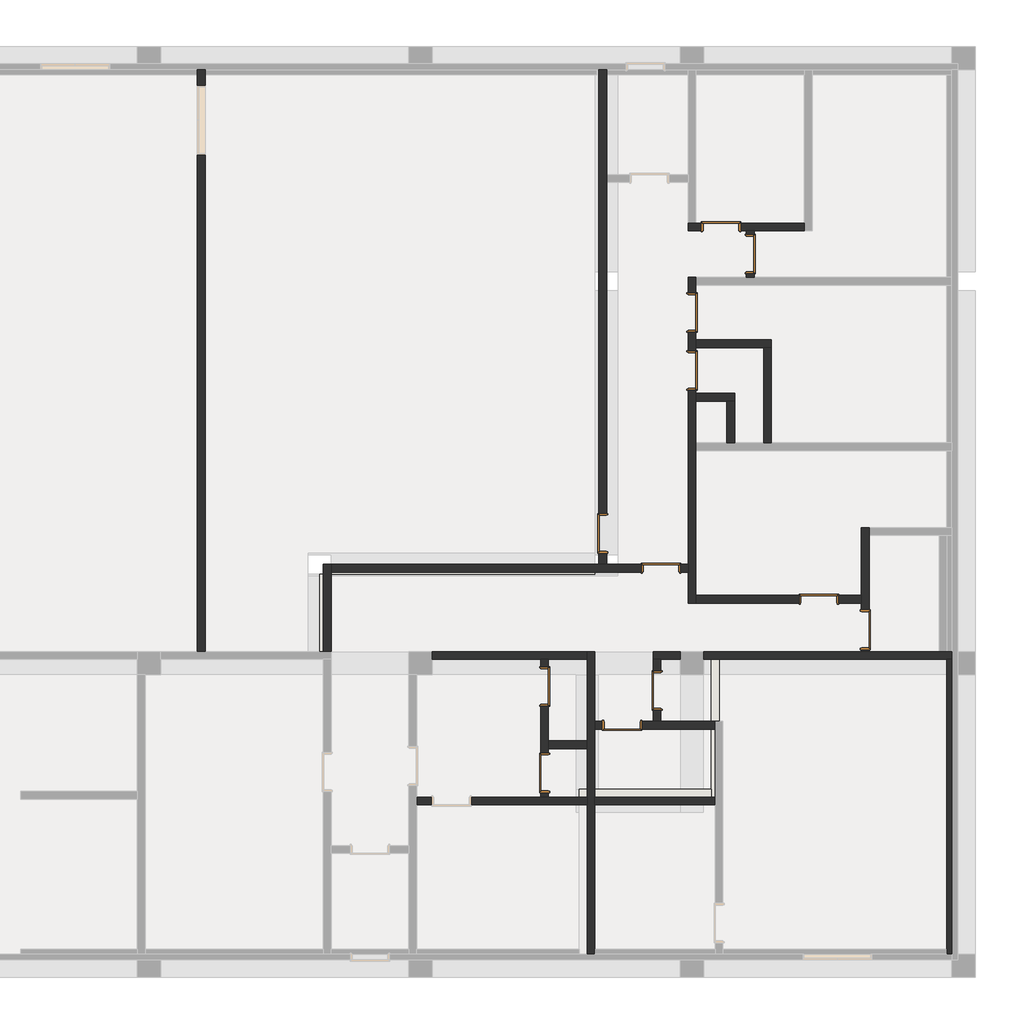
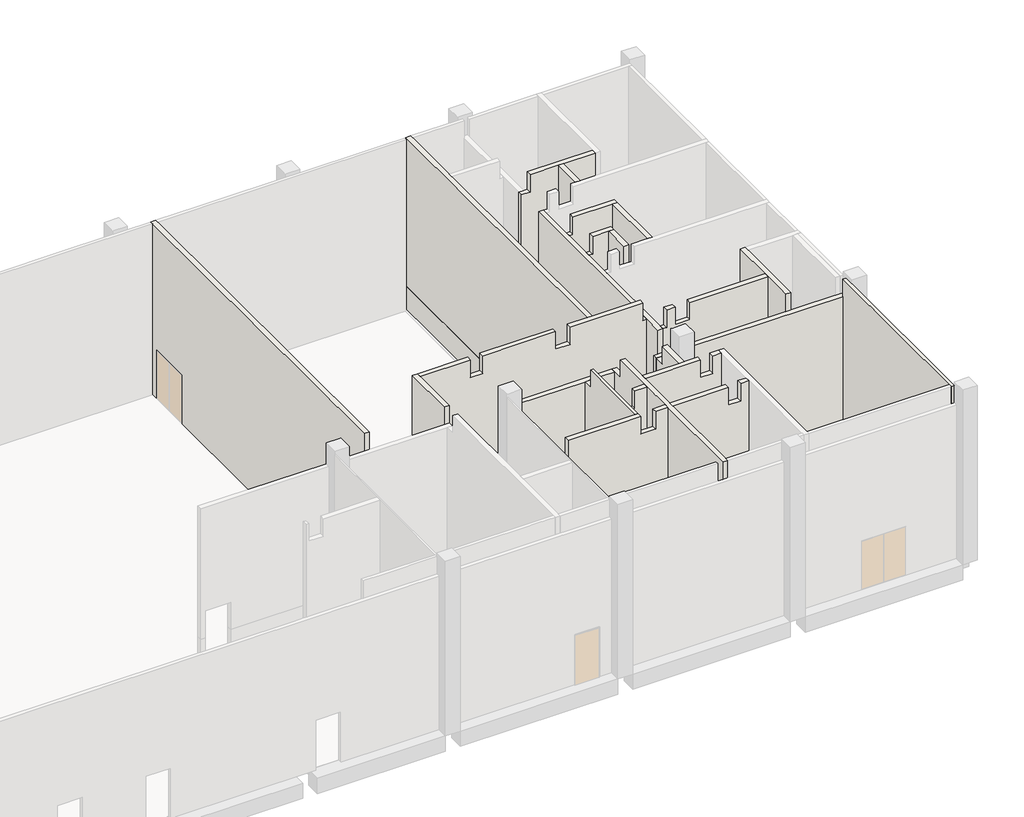
# One storey, part 2 of 4: 29 walls, 12 doors.
# Revit data of these elements (continued)
# Elements 19, 20, 21, 22, 23, 24, 25, 26, 27, 28, 29, 30, 31, 32, 33, 34, 35, 36, 37, 38, 39, 40 (IfcWall, "H_WA_AR B02_Int Wall MA_IW1 T200") (continued)
#   Base Offset = 0 mm
#   wall height = 7500.038 mm
#   H_Wall Style No = IW211_BL
#   Phase Created = New Construction
#   Base Constraint = TOC(GF)
#   Top Constraint = TOC
#   Materials on its faces: "00_Masonry_Conc. Block"
# Element 41 (IfcWall, "H_WA_AR B02_Ext Wall DY-IN_EW1_VB")
#   Top Offset = 0 mm
#   Base Offset = 0 mm
#   wall height = 7500.038 mm
#   Phase Created = New Construction
#   Base Constraint = TOC(GF)
#   Top Constraint = TOC
#   Materials on its faces: "Rock Wool"
# Materials
#   "00_Masonry_Conc. Block": class "Concrete", colour RGB 180 180 180, transparency 0, Description = "Conc. Block", Cost = 0, Image = Brick_Uniform_12inch_Running_Gray.png
#   "Rock Wool": class "Generic", colour RGB 120 120 120, transparency 0, Description = "Rock Wool", Cost = 0
#   "00_Concrete_Reinf. Conc.": class "Concrete", colour RGB 176 176 176, transparency 0, Description = "Reinf. Conc.", Cost = 0, Image = Concrete.Cast-In-Place.Flat.Polished.Grey.jpg
